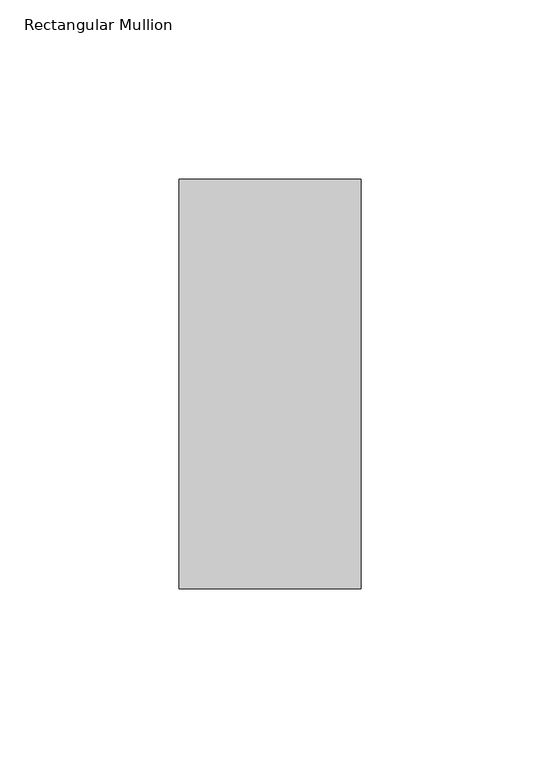
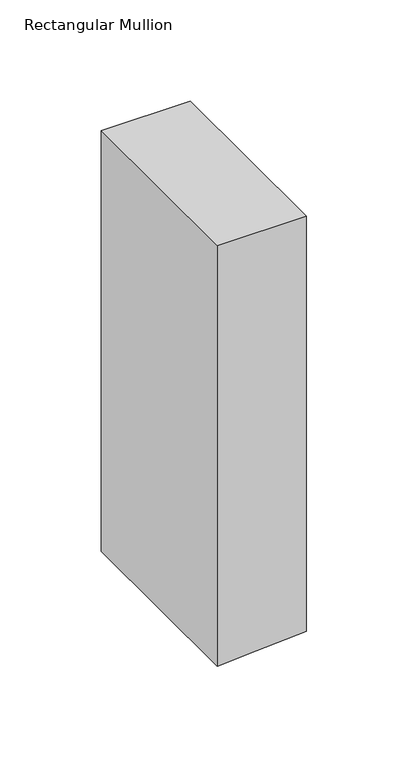
"""IFC4 building model written with IfcOpenShell, lengths in millimetres: member geometry, Rectangular Mullion : KAWNEER TRIFAB VERSAGLAZE 451T - CLEAR ANODIZED ALUM. - BACK GLAZED."""

import ifcopenshell
import ifcopenshell.guid

model = None  # the IFC model being written
_history = None  # IfcOwnerHistory: only IFC2X3 demands one
_inside = {}  # id of a spatial element -> (the spatial element, [elements in it])
_under = {}  # id of a project, library or spatial element -> (it, [spatial elements below it])
_declared = {}  # id of a project -> (the project, [libraries it declares])
_typed = {}  # id of a type object -> (the type object, [elements of that type])
_made_of = {}  # id of a material, layer set ... -> (it, [elements and type objects made of it])


def new_model(schema):
    """Start an empty IFC model of exactly this schema.

    Asked for "IFC4X3", IfcOpenShell would pick the latest addendum, in which some entities
    have other attributes; the version numbers below select the first issue.
    IFC2X3 requires an IfcOwnerHistory on every rooted entity: one is made here for all.
    """
    global model, _history
    if schema == "IFC4X3":
        model = ifcopenshell.file(schema_version=(4, 3, 0, 0))
    else:
        model = ifcopenshell.file(schema=schema)
    _inside.clear()
    _under.clear()
    _declared.clear()
    _typed.clear()
    _made_of.clear()
    _history = None
    if model.schema == "IFC2X3":
        org = make("IfcOrganization", Name="unknown")
        user = make(
            "IfcPersonAndOrganization",
            ThePerson=make("IfcPerson", FamilyName="unknown"),
            TheOrganization=org,
        )
        app = make(
            "IfcApplication",
            ApplicationDeveloper=org,
            Version="unknown",
            ApplicationFullName="unknown",
            ApplicationIdentifier="unknown",
        )
        _history = make(
            "IfcOwnerHistory",
            OwningUser=user,
            OwningApplication=app,
            ChangeAction="ADDED",
            CreationDate=0,
        )
    return model


def make(cls, **values):
    """One entity of the class cls with the attributes given. An attribute that is None is left unset."""
    return model.create_entity(
        cls, **{name: value for name, value in values.items() if value is not None}
    )


def rooted(cls, **values):
    """An entity with a GlobalId (a new one), such as an element, a storey or a relation."""
    return make(cls, GlobalId=ifcopenshell.guid.new(), OwnerHistory=_history, **values)


def si_unit(unit_type, name, prefix=None):
    """IfcSIUnit, for example si_unit("LENGTHUNIT", "METRE", prefix="MILLI")."""
    return make("IfcSIUnit", UnitType=unit_type, Prefix=prefix, Name=name)


def assignment(units):
    """IfcUnitAssignment: the units of a project."""
    return None if units is None else make("IfcUnitAssignment", Units=units)


def point(xyz):
    """IfcCartesianPoint."""
    return None if xyz is None else make("IfcCartesianPoint", Coordinates=xyz)


def direction(xyz):
    """IfcDirection."""
    return None if xyz is None else make("IfcDirection", DirectionRatios=xyz)


def frame(location, z_axis=None, x_axis=None):
    """IfcAxis2Placement3D, a coordinate frame: its origin and axes. An axis left out is left unset."""
    return make(
        "IfcAxis2Placement3D",
        Location=point(location),
        Axis=direction(z_axis),
        RefDirection=direction(x_axis),
    )


def origin():
    """The frame at (0, 0, 0) with its axes left unset."""
    return frame((0.0, 0.0, 0.0))


def place(relative_to, where):
    """IfcLocalPlacement: puts the frame where relative to a parent placement (None: the world)."""
    return make(
        "IfcLocalPlacement", PlacementRelTo=relative_to, RelativePlacement=where
    )


def context(
    kind, dimensions, precision=None, world=None, true_north=None, identifier=None
):
    """IfcGeometricRepresentationContext, for example the 3D "Model" context."""
    return make(
        "IfcGeometricRepresentationContext",
        ContextIdentifier=identifier,
        ContextType=kind,
        CoordinateSpaceDimension=dimensions,
        Precision=precision,
        WorldCoordinateSystem=world,
        TrueNorth=true_north,
    )


def project(units=None, contexts=None):
    """IfcProject with its units and contexts."""
    return rooted(
        "IfcProject",
        Name="project",
        RepresentationContexts=contexts,
        UnitsInContext=assignment(units),
    )


def spatial(cls, under=None, at=None, **own):
    """A site, building, storey or space (cls), placed at a placement, below another one or the project."""
    s = rooted(cls, ObjectPlacement=at, **own)
    if under is not None:
        _under.setdefault(under.id(), (under, []))[1].append(s)
    return s


def polyline(points):
    """IfcPolyline through the points."""
    return make("IfcPolyline", Points=[point(p) for p in points])


def outline(outer, holes=None, kind="AREA"):
    """IfcArbitraryClosedProfileDef: a profile drawn as a closed curve; with holes, ...WithVoids."""
    if holes is None:
        return make("IfcArbitraryClosedProfileDef", ProfileType=kind, OuterCurve=outer)
    return make(
        "IfcArbitraryProfileDefWithVoids",
        ProfileType=kind,
        OuterCurve=outer,
        InnerCurves=holes,
    )


def extrude(swept, where, along, depth):
    """IfcExtrudedAreaSolid: the profile swept, set in the frame where, extruded along a direction by depth."""
    return make(
        "IfcExtrudedAreaSolid",
        SweptArea=swept,
        Position=where,
        ExtrudedDirection=direction(along),
        Depth=depth,
    )


def shape(context_of_items, identifier, shape_type, items):
    """IfcShapeRepresentation: the items that make up one representation, for example the "Body"."""
    return make(
        "IfcShapeRepresentation",
        ContextOfItems=context_of_items,
        RepresentationIdentifier=identifier,
        RepresentationType=shape_type,
        Items=items,
    )


def source(mapping_origin, context_of_items, identifier, shape_type, items):
    """IfcRepresentationMap: a shape defined once, which mapped items show again and again."""
    return make(
        "IfcRepresentationMap",
        MappingOrigin=mapping_origin,
        MappedRepresentation=shape(context_of_items, identifier, shape_type, items),
    )


def transform(
    local_origin,
    x_axis=None,
    y_axis=None,
    z_axis=None,
    scale=None,
    scale2=None,
    scale3=None,
    uniform=True,
):
    """IfcCartesianTransformationOperator3D, or its non-uniform kind. x_axis, y_axis, z_axis: its Axis1, 2, 3."""
    if uniform:
        return make(
            "IfcCartesianTransformationOperator3D",
            Axis1=direction(x_axis),
            Axis2=direction(y_axis),
            LocalOrigin=point(local_origin),
            Scale=scale,
            Axis3=direction(z_axis),
        )
    return make(
        "IfcCartesianTransformationOperator3DnonUniform",
        Axis1=direction(x_axis),
        Axis2=direction(y_axis),
        LocalOrigin=point(local_origin),
        Scale=scale,
        Axis3=direction(z_axis),
        Scale2=scale2,
        Scale3=scale3,
    )


def mapped(mapping_source, mapping_target):
    """IfcMappedItem: shows the shape of a source again, moved by a transform."""
    return make(
        "IfcMappedItem", MappingSource=mapping_source, MappingTarget=mapping_target
    )


def made_of(thing, what):
    """Note that an element or type object is made of a material, layer set ...; save() writes the relation."""
    if what is not None:
        _made_of.setdefault(what.id(), (what, []))[1].append(thing)
    return thing


def element(
    cls,
    number,
    at=None,
    inside=None,
    cuts=None,
    type_object=None,
    material=None,
    context=None,
    identifier="Body",
    shape_type=None,
    held_by="IfcProductDefinitionShape",
    body=None,
    shapes=None,
    **own,
):
    """One element of the class cls, such as IfcWall. Its Tag is "e" and its number.

    at: its placement. inside: the storey or other place that contains it. cuts: it is an
    opening in that element (IfcRelVoidsElement). A single representation is given by context,
    identifier, shape_type and body (its items); several are given by shapes. held_by: the class
    of the entity that holds the representations. save() writes the other relations.
    """
    e = rooted(cls, Tag="e%d" % number, ObjectPlacement=at, **own)
    if body is not None:
        shapes = [shape(context, identifier, shape_type, body)]
    if shapes is not None:
        e.Representation = make(held_by, Representations=shapes)
    if inside is not None:
        _inside.setdefault(inside.id(), (inside, []))[1].append(e)
    if cuts is not None:
        rooted(
            "IfcRelVoidsElement", RelatingBuildingElement=cuts, RelatedOpeningElement=e
        )
    if type_object is not None:
        _typed.setdefault(type_object.id(), (type_object, []))[1].append(e)
    return made_of(e, material)


def aggregate(whole, parts):
    """IfcRelAggregates: a whole, such as a stair, and the parts it consists of."""
    return rooted("IfcRelAggregates", RelatingObject=whole, RelatedObjects=parts)


def save(model, path):
    """Write the relations noted so far, then the file.

    IfcRelAggregates (storeys below a building ...), IfcRelContainedInSpatialStructure (elements
    in a storey), IfcRelDefinesByType, IfcRelAssociatesMaterial and IfcRelDeclares: one each for
    every whole, place, type object, material and project.
    """
    for whole, parts in _under.values():
        aggregate(whole, parts)
    for where, things in _inside.values():
        rooted(
            "IfcRelContainedInSpatialStructure",
            RelatedElements=things,
            RelatingStructure=where,
        )
    for kind, things in _typed.values():
        rooted("IfcRelDefinesByType", RelatedObjects=things, RelatingType=kind)
    for what, things in _made_of.values():
        rooted("IfcRelAssociatesMaterial", RelatedObjects=things, RelatingMaterial=what)
    for by, libraries in _declared.values():
        rooted("IfcRelDeclares", RelatingContext=by, RelatedDefinitions=libraries)
    model.write(path)


def rectangular_mullion_f1e3b744(model_context):
    return source(origin(), model_context, "Body", "SweptSolid", [
        extrude(outline(polyline([(0.0, 25.4), (0.0, -25.4), (-253.4747345, -25.4), (-252.0852855, -3.1688169), (-250.2997345, 25.4), (0.0, 25.4)])), frame((0.0, -57.15, 0.0), z_axis=(0.0, 1.0, 0.0), x_axis=(0.0, 0.0, 1.0)), (0.0, 0.0, 1.0), 114.3),
    ])


if __name__ == "__main__":
    model = new_model("IFC4")
    model_context = context("Model", 3, world=origin())
    ifc_project = project(units=[si_unit("LENGTHUNIT", "METRE", prefix="MILLI")], contexts=[model_context])
    site = spatial("IfcSite", under=ifc_project)
    building = spatial("IfcBuilding", under=site)
    placement = place(None, origin())
    rectangular_mullion_shape = rectangular_mullion_f1e3b744(model_context)
    element("IfcMember", 1, ObjectType="Rectangular Mullion : KAWNEER TRIFAB VERSAGLAZE 451T - CLEAR ANODIZED ALUM. - BACK GLAZED", at=placement, inside=building, context=model_context, shape_type="MappedRepresentation", body=[
        mapped(rectangular_mullion_shape, transform((0.0, 0.0, 0.0), x_axis=(1.0, 0.0, 0.0), y_axis=(0.0, 1.0, 0.0), z_axis=(0.0, 0.0, 1.0))),
    ])
    save(model, "model.ifc")

# Revit data of these elements
# Type "Rectangular Mullion : KAWNEER TRIFAB VERSAGLAZE 451T - CLEAR ANODIZED ALUM. - BACK GLAZED"
#   built-in parameter 1007304 = 0.375 (stored number, unit not read)
#   built-in parameter 1007301 = 0.0833333 (stored number, unit not read)
#   built-in parameter 1007300 = 0.0833333 (stored number, unit not read)
# Element 1 (IfcMember, "Rectangular Mullion : KAWNEER TRIFAB VERSAGLAZE 451T - CLEAR ANODIZED ALUM. - BACK GLAZED")
#   Materials on its faces: "KAWNEER TRIFAB VERSAGLAZE 451T - CLEAR ANODIZED ALUM. - BACK GLAZED"
# Materials
#   "KAWNEER TRIFAB VERSAGLAZE 451T - CLEAR ANODIZED ALUM. - BACK GLAZED": class "Metal", colour RGB 244 244 244, transparency 0, Description = "Aluminum 6061", Cost = 0
